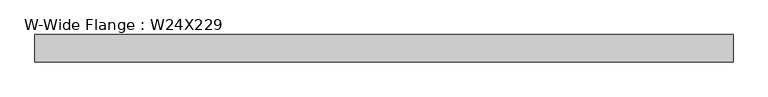
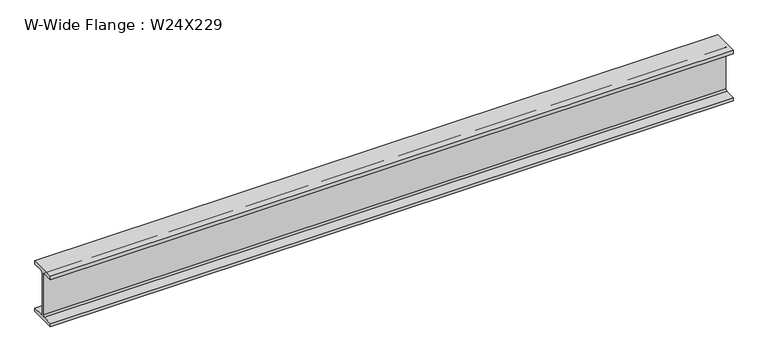
"""IFC4 building model written with IfcOpenShell, lengths in millimetres: beam geometry, W-Wide Flange : W24X229."""

from ifc_helpers import new_model, si_unit, point, frame, frame_2d, origin, place, context, project, spatial, polyline, circle_curve, trimmed, segment, composite_curve, outline, extrude, source, transform, mapped, element, save


def w_wide_flange_w24x229_264a0a21(model_context):
    return source(origin(), model_context, "Body", "SweptSolid", [
        extrude(outline(composite_curve([segment(polyline([(166.37, -286.258), (166.37, -330.2), (-166.37, -330.2), (-166.37, -286.258), (-34.925, -286.258)]), True, "CONTINUOUS"), segment(trimmed(circle_curve(frame_2d((-34.925, -263.525)), 22.733), [point((-34.925, -286.258))], [point((-12.192, -263.525))], True, "CARTESIAN"), True, "CONTINUOUS"), segment(polyline([(-12.192, -263.525), (-12.192, 263.525)]), True, "CONTINUOUS"), segment(trimmed(circle_curve(frame_2d((-34.925, 263.525)), 22.733), [point((-12.192, 263.525))], [point((-34.925, 286.258))], True, "CARTESIAN"), True, "CONTINUOUS"), segment(polyline([(-34.925, 286.258), (-166.37, 286.258), (-166.37, 330.2), (166.37, 330.2), (166.37, 286.258), (34.925, 286.258)]), True, "CONTINUOUS"), segment(trimmed(circle_curve(frame_2d((34.925, 263.525)), 22.733), [point((34.925, 286.258))], [point((12.192, 263.525))], True, "CARTESIAN"), True, "CONTINUOUS"), segment(polyline([(12.192, 263.525), (12.192, -263.525)]), True, "CONTINUOUS"), segment(trimmed(circle_curve(frame_2d((34.925, -263.525)), 22.733), [point((12.192, -263.525))], [point((34.925, -286.258))], True, "CARTESIAN"), True, "CONTINUOUS"), segment(polyline([(34.925, -286.258), (166.37, -286.258)]), True, "CONTINUOUS")], self_intersect=False)), frame((-4220.21, 0.0, 0.0), z_axis=(1.0, 0.0, 0.0), x_axis=(0.0, 1.0, 0.0)), (0.0, 0.0, 1.0), 8440.42),
    ])


if __name__ == "__main__":
    model = new_model("IFC4")
    model_context = context("Model", 3, world=origin())
    ifc_project = project(units=[si_unit("LENGTHUNIT", "METRE", prefix="MILLI")], contexts=[model_context])
    site = spatial("IfcSite", under=ifc_project)
    building = spatial("IfcBuilding", under=site)
    placement = place(None, origin())
    w_wide_flange_w24x229_shape = w_wide_flange_w24x229_264a0a21(model_context)
    element("IfcBeam", 1, ObjectType="W-Wide Flange : W24X229", at=placement, inside=building, context=model_context, shape_type="MappedRepresentation", body=[
        mapped(w_wide_flange_w24x229_shape, transform((0.0, 0.0, 0.0), x_axis=(1.0, 0.0, 0.0), y_axis=(0.0, 1.0, 0.0), z_axis=(0.0, 0.0, 1.0))),
    ])
    save(model, "model.ifc")

# Revit data of these elements
# Type "W-Wide Flange : W24X229"
#   Assembly Code = "B10"
#   W = 229
#   Start Extension Calculation [instance default] = 10' - 0"
#   Start Extension [instance default] = -0' - 0 1/2"
#   End Extension Calculation [instance default] = 10' - 0"
#   End Extension [instance default] = -0' - 0 1/2"
#   Length [instance default] = 5' - 0"
#   bf = 1' - 1.1"
#   d = 2' - 2"
#   k = 0' - 2 5/8"
#   k2 = 0' - 0.895"
#   tf = 0' - 1.73"
#   tw = 0' - 0.96"
#   A = 0.466667 SF
#   Beam Material [instance default] = Metal - Steel - ASTM A992
# Element 1 (IfcBeam, "W-Wide Flange : W24X229")
#   Materials on its faces: "Metal - Steel - ASTM A992"
# Materials
#   "Metal - Steel - ASTM A992": class "Metal", colour RGB 128 0 0, transparency 0
